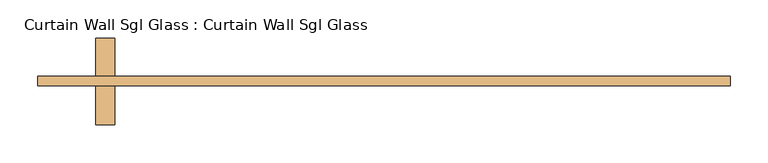
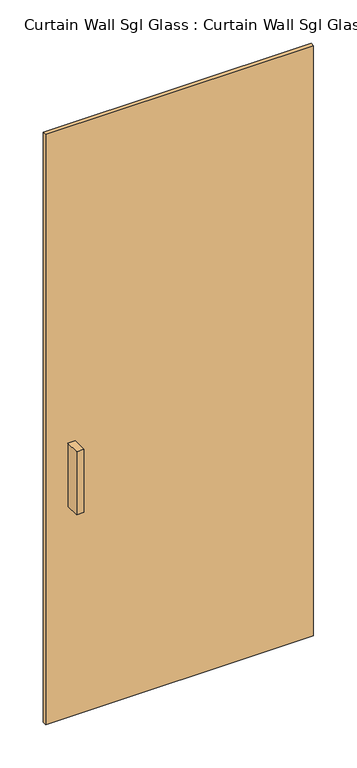
"""IFC4 building model written with IfcOpenShell, lengths in millimetres: door geometry, Curtain Wall Sgl Glass : Curtain Wall Sgl Glass."""

from ifc_helpers import new_model, si_unit, frame, origin, origin_with_axes, place, context, project, spatial, polyline, outline, extrude, source, transform, mapped, element, save


def curtain_wall_sgl_glass_curtain_wall_sgl_glass_c2d4b377(model_context):
    return source(origin(), model_context, "Body", "SweptSolid", [
        extrude(outline(polyline([(-355.6, 12.7), (-355.6, -38.1), (-381.0, -38.1), (-381.0, 12.7), (-355.6, 12.7)])), frame((0.0, 0.0, 762.0), z_axis=(0.0, 0.0, 1.0), x_axis=(1.0, 0.0, 0.0)), (0.0, 0.0, 1.0), 228.6),
        extrude(outline(polyline([(-381.0, -101.6), (-381.0, -50.8), (-355.6, -50.8), (-355.6, -101.6), (-381.0, -101.6)])), frame((0.0, 0.0, 762.0), z_axis=(0.0, 0.0, 1.0), x_axis=(1.0, 0.0, 0.0)), (0.0, 0.0, 1.0), 228.6),
        extrude(outline(polyline([(457.2, -50.8), (-457.2, -50.8), (-457.2, -38.1), (457.2, -38.1), (457.2, -50.8)])), origin_with_axes(), (0.0, 0.0, 1.0), 2133.6),
    ])


if __name__ == "__main__":
    model = new_model("IFC4")
    model_context = context("Model", 3, world=origin())
    ifc_project = project(units=[si_unit("LENGTHUNIT", "METRE", prefix="MILLI")], contexts=[model_context])
    site = spatial("IfcSite", under=ifc_project)
    building = spatial("IfcBuilding", under=site)
    placement = place(None, origin())
    curtain_wall_sgl_glass_curtain_wall_sgl_glass_shape = curtain_wall_sgl_glass_curtain_wall_sgl_glass_c2d4b377(model_context)
    element("IfcDoor", 1, ObjectType="Curtain Wall Sgl Glass : Curtain Wall Sgl Glass", at=placement, inside=building, context=model_context, shape_type="MappedRepresentation", body=[
        mapped(curtain_wall_sgl_glass_curtain_wall_sgl_glass_shape, transform((0.0, 0.0, 0.0), x_axis=(1.0, 0.0, 0.0), y_axis=(0.0, 1.0, 0.0), z_axis=(0.0, 0.0, 1.0))),
    ])
    save(model, "model.ifc")

# Revit data of these elements
# Type "Curtain Wall Sgl Glass : Curtain Wall Sgl Glass"
#   Assembly Code = "B2030100"
#   Offset = 0' - 2"
#   Function = 1
#   Handle Material = Metal - Aluminum
#   Glazing Material = Glass
# Element 1 (IfcDoor, "Curtain Wall Sgl Glass : Curtain Wall Sgl Glass")
#   Materials on its faces: "Metal - Aluminum", "Glass"
# Materials
#   "Metal - Aluminum": class "Metal", colour RGB 140 140 140, transparency 0, Cost = 0
#   "Glass": class "Glass", colour RGB 0 128 192, transparency 0.75, Cost = 0
